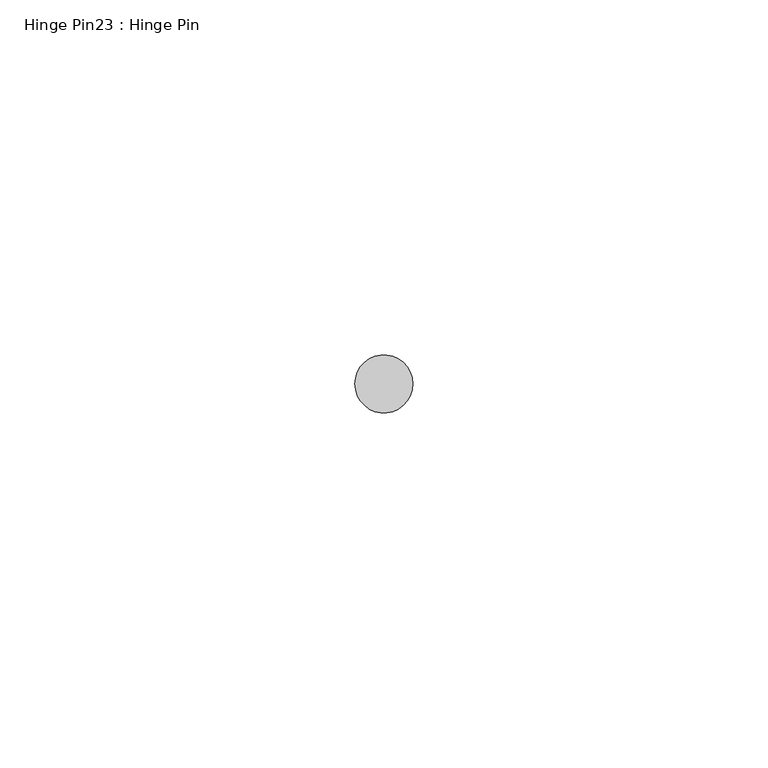
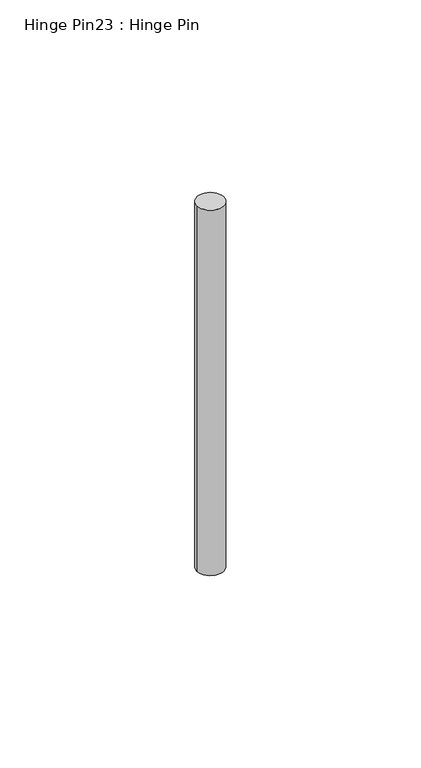
"""IFC4 building model written with IfcOpenShell, lengths in millimetres: proxy geometry, Hinge Pin23 : Hinge Pin."""

import ifcopenshell
import ifcopenshell.guid

model = None  # the IFC model being written
_history = None  # IfcOwnerHistory: only IFC2X3 demands one
_inside = {}  # id of a spatial element -> (the spatial element, [elements in it])
_under = {}  # id of a project, library or spatial element -> (it, [spatial elements below it])
_declared = {}  # id of a project -> (the project, [libraries it declares])
_typed = {}  # id of a type object -> (the type object, [elements of that type])
_made_of = {}  # id of a material, layer set ... -> (it, [elements and type objects made of it])


def new_model(schema):
    """Start an empty IFC model of exactly this schema.

    Asked for "IFC4X3", IfcOpenShell would pick the latest addendum, in which some entities
    have other attributes; the version numbers below select the first issue.
    IFC2X3 requires an IfcOwnerHistory on every rooted entity: one is made here for all.
    """
    global model, _history
    if schema == "IFC4X3":
        model = ifcopenshell.file(schema_version=(4, 3, 0, 0))
    else:
        model = ifcopenshell.file(schema=schema)
    _inside.clear()
    _under.clear()
    _declared.clear()
    _typed.clear()
    _made_of.clear()
    _history = None
    if model.schema == "IFC2X3":
        org = make("IfcOrganization", Name="unknown")
        user = make(
            "IfcPersonAndOrganization",
            ThePerson=make("IfcPerson", FamilyName="unknown"),
            TheOrganization=org,
        )
        app = make(
            "IfcApplication",
            ApplicationDeveloper=org,
            Version="unknown",
            ApplicationFullName="unknown",
            ApplicationIdentifier="unknown",
        )
        _history = make(
            "IfcOwnerHistory",
            OwningUser=user,
            OwningApplication=app,
            ChangeAction="ADDED",
            CreationDate=0,
        )
    return model


def make(cls, **values):
    """One entity of the class cls with the attributes given. An attribute that is None is left unset."""
    return model.create_entity(
        cls, **{name: value for name, value in values.items() if value is not None}
    )


def rooted(cls, **values):
    """An entity with a GlobalId (a new one), such as an element, a storey or a relation."""
    return make(cls, GlobalId=ifcopenshell.guid.new(), OwnerHistory=_history, **values)


def si_unit(unit_type, name, prefix=None):
    """IfcSIUnit, for example si_unit("LENGTHUNIT", "METRE", prefix="MILLI")."""
    return make("IfcSIUnit", UnitType=unit_type, Prefix=prefix, Name=name)


def assignment(units):
    """IfcUnitAssignment: the units of a project."""
    return None if units is None else make("IfcUnitAssignment", Units=units)


def point(xyz):
    """IfcCartesianPoint."""
    return None if xyz is None else make("IfcCartesianPoint", Coordinates=xyz)


def direction(xyz):
    """IfcDirection."""
    return None if xyz is None else make("IfcDirection", DirectionRatios=xyz)


def frame(location, z_axis=None, x_axis=None):
    """IfcAxis2Placement3D, a coordinate frame: its origin and axes. An axis left out is left unset."""
    return make(
        "IfcAxis2Placement3D",
        Location=point(location),
        Axis=direction(z_axis),
        RefDirection=direction(x_axis),
    )


def frame_2d(location, x_axis=None):
    """IfcAxis2Placement2D, a coordinate frame in the plane: its origin and x axis."""
    return make(
        "IfcAxis2Placement2D", Location=point(location), RefDirection=direction(x_axis)
    )


def origin():
    """The frame at (0, 0, 0) with its axes left unset."""
    return frame((0.0, 0.0, 0.0))


def place(relative_to, where):
    """IfcLocalPlacement: puts the frame where relative to a parent placement (None: the world)."""
    return make(
        "IfcLocalPlacement", PlacementRelTo=relative_to, RelativePlacement=where
    )


def context(
    kind, dimensions, precision=None, world=None, true_north=None, identifier=None
):
    """IfcGeometricRepresentationContext, for example the 3D "Model" context."""
    return make(
        "IfcGeometricRepresentationContext",
        ContextIdentifier=identifier,
        ContextType=kind,
        CoordinateSpaceDimension=dimensions,
        Precision=precision,
        WorldCoordinateSystem=world,
        TrueNorth=true_north,
    )


def project(units=None, contexts=None):
    """IfcProject with its units and contexts."""
    return rooted(
        "IfcProject",
        Name="project",
        RepresentationContexts=contexts,
        UnitsInContext=assignment(units),
    )


def spatial(cls, under=None, at=None, **own):
    """A site, building, storey or space (cls), placed at a placement, below another one or the project."""
    s = rooted(cls, ObjectPlacement=at, **own)
    if under is not None:
        _under.setdefault(under.id(), (under, []))[1].append(s)
    return s


def circle_curve(where, radius):
    """IfcCircle in the frame where."""
    return make("IfcCircle", Position=where, Radius=radius)


def trimmed(basis, trim1, trim2, sense, master):
    """IfcTrimmedCurve: the piece of a basis curve between two trims."""
    return make(
        "IfcTrimmedCurve",
        BasisCurve=basis,
        Trim1=trim1,
        Trim2=trim2,
        SenseAgreement=sense,
        MasterRepresentation=master,
    )


def segment(curve, same_sense, transition):
    """IfcCompositeCurveSegment."""
    return make(
        "IfcCompositeCurveSegment",
        Transition=transition,
        SameSense=same_sense,
        ParentCurve=curve,
    )


def composite_curve(segments, self_intersect=None):
    """IfcCompositeCurve: segments joined end to end."""
    return make("IfcCompositeCurve", Segments=segments, SelfIntersect=self_intersect)


def outline(outer, holes=None, kind="AREA"):
    """IfcArbitraryClosedProfileDef: a profile drawn as a closed curve; with holes, ...WithVoids."""
    if holes is None:
        return make("IfcArbitraryClosedProfileDef", ProfileType=kind, OuterCurve=outer)
    return make(
        "IfcArbitraryProfileDefWithVoids",
        ProfileType=kind,
        OuterCurve=outer,
        InnerCurves=holes,
    )


def extrude(swept, where, along, depth):
    """IfcExtrudedAreaSolid: the profile swept, set in the frame where, extruded along a direction by depth."""
    return make(
        "IfcExtrudedAreaSolid",
        SweptArea=swept,
        Position=where,
        ExtrudedDirection=direction(along),
        Depth=depth,
    )


def shape(context_of_items, identifier, shape_type, items):
    """IfcShapeRepresentation: the items that make up one representation, for example the "Body"."""
    return make(
        "IfcShapeRepresentation",
        ContextOfItems=context_of_items,
        RepresentationIdentifier=identifier,
        RepresentationType=shape_type,
        Items=items,
    )


def source(mapping_origin, context_of_items, identifier, shape_type, items):
    """IfcRepresentationMap: a shape defined once, which mapped items show again and again."""
    return make(
        "IfcRepresentationMap",
        MappingOrigin=mapping_origin,
        MappedRepresentation=shape(context_of_items, identifier, shape_type, items),
    )


def transform(
    local_origin,
    x_axis=None,
    y_axis=None,
    z_axis=None,
    scale=None,
    scale2=None,
    scale3=None,
    uniform=True,
):
    """IfcCartesianTransformationOperator3D, or its non-uniform kind. x_axis, y_axis, z_axis: its Axis1, 2, 3."""
    if uniform:
        return make(
            "IfcCartesianTransformationOperator3D",
            Axis1=direction(x_axis),
            Axis2=direction(y_axis),
            LocalOrigin=point(local_origin),
            Scale=scale,
            Axis3=direction(z_axis),
        )
    return make(
        "IfcCartesianTransformationOperator3DnonUniform",
        Axis1=direction(x_axis),
        Axis2=direction(y_axis),
        LocalOrigin=point(local_origin),
        Scale=scale,
        Axis3=direction(z_axis),
        Scale2=scale2,
        Scale3=scale3,
    )


def mapped(mapping_source, mapping_target):
    """IfcMappedItem: shows the shape of a source again, moved by a transform."""
    return make(
        "IfcMappedItem", MappingSource=mapping_source, MappingTarget=mapping_target
    )


def made_of(thing, what):
    """Note that an element or type object is made of a material, layer set ...; save() writes the relation."""
    if what is not None:
        _made_of.setdefault(what.id(), (what, []))[1].append(thing)
    return thing


def element(
    cls,
    number,
    at=None,
    inside=None,
    cuts=None,
    type_object=None,
    material=None,
    context=None,
    identifier="Body",
    shape_type=None,
    held_by="IfcProductDefinitionShape",
    body=None,
    shapes=None,
    **own,
):
    """One element of the class cls, such as IfcWall. Its Tag is "e" and its number.

    at: its placement. inside: the storey or other place that contains it. cuts: it is an
    opening in that element (IfcRelVoidsElement). A single representation is given by context,
    identifier, shape_type and body (its items); several are given by shapes. held_by: the class
    of the entity that holds the representations. save() writes the other relations.
    """
    e = rooted(cls, Tag="e%d" % number, ObjectPlacement=at, **own)
    if body is not None:
        shapes = [shape(context, identifier, shape_type, body)]
    if shapes is not None:
        e.Representation = make(held_by, Representations=shapes)
    if inside is not None:
        _inside.setdefault(inside.id(), (inside, []))[1].append(e)
    if cuts is not None:
        rooted(
            "IfcRelVoidsElement", RelatingBuildingElement=cuts, RelatedOpeningElement=e
        )
    if type_object is not None:
        _typed.setdefault(type_object.id(), (type_object, []))[1].append(e)
    return made_of(e, material)


def aggregate(whole, parts):
    """IfcRelAggregates: a whole, such as a stair, and the parts it consists of."""
    return rooted("IfcRelAggregates", RelatingObject=whole, RelatedObjects=parts)


def save(model, path):
    """Write the relations noted so far, then the file.

    IfcRelAggregates (storeys below a building ...), IfcRelContainedInSpatialStructure (elements
    in a storey), IfcRelDefinesByType, IfcRelAssociatesMaterial and IfcRelDeclares: one each for
    every whole, place, type object, material and project.
    """
    for whole, parts in _under.values():
        aggregate(whole, parts)
    for where, things in _inside.values():
        rooted(
            "IfcRelContainedInSpatialStructure",
            RelatedElements=things,
            RelatingStructure=where,
        )
    for kind, things in _typed.values():
        rooted("IfcRelDefinesByType", RelatedObjects=things, RelatingType=kind)
    for what, things in _made_of.values():
        rooted("IfcRelAssociatesMaterial", RelatedObjects=things, RelatingMaterial=what)
    for by, libraries in _declared.values():
        rooted("IfcRelDeclares", RelatingContext=by, RelatedDefinitions=libraries)
    model.write(path)


def hinge_pin23_hinge_pin_2f9686dc(model_context):
    return source(origin(), model_context, "Body", "SweptSolid", [
        extrude(outline(composite_curve([segment(trimmed(circle_curve(frame_2d((587319.1320739, -536310.3652841)), 4.0894), [point((587315.0426739, -536310.3652841))], [point((587323.2214739, -536310.3652841))], False, "CARTESIAN"), True, "CONTINUOUS"), segment(trimmed(circle_curve(frame_2d((587319.1320739, -536310.3652841)), 4.0894), [point((587323.2214739, -536310.3652841))], [point((587315.0426739, -536310.3652841))], False, "CARTESIAN"), True, "CONTINUOUS")], self_intersect=False)), frame((0.0, 0.0, 1128.5140625), z_axis=(0.0, 0.0, 1.0), x_axis=(1.0, 0.0, 0.0)), (0.0, 0.0, 1.0), 117.871875),
    ])


if __name__ == "__main__":
    model = new_model("IFC4")
    model_context = context("Model", 3, world=origin())
    ifc_project = project(units=[si_unit("LENGTHUNIT", "METRE", prefix="MILLI")], contexts=[model_context])
    site = spatial("IfcSite", under=ifc_project)
    building = spatial("IfcBuilding", under=site)
    placement = place(None, origin())
    hinge_pin23_hinge_pin_shape = hinge_pin23_hinge_pin_2f9686dc(model_context)
    element("IfcBuildingElementProxy", 1, Name="Hinge Pin23 : Hinge Pin", ObjectType="Hinge Pin23 : Hinge Pin", at=placement, inside=building, context=model_context, shape_type="MappedRepresentation", body=[
        mapped(hinge_pin23_hinge_pin_shape, transform((0.0, 0.0, 0.0), x_axis=(1.0, 0.0, 0.0), y_axis=(0.0, 1.0, 0.0), z_axis=(0.0, 0.0, 1.0))),
    ])
    save(model, "model.ifc")

# Revit data of these elements
# Element 1 (IfcBuildingElementProxy, "Hinge Pin23 : Hinge Pin")
#   Materials on its faces: "6\"X6\" WELD-ON STL BUTT HINGE"
# Materials
#   "6\"X6\" WELD-ON STL BUTT HINGE": class "Metal", colour RGB 189 187 185, transparency 0, Description = "Carbon steel", Cost = 0
